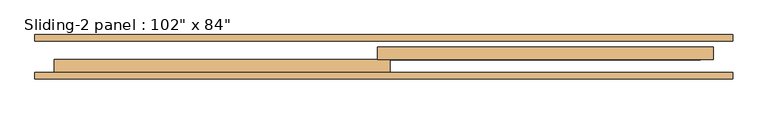
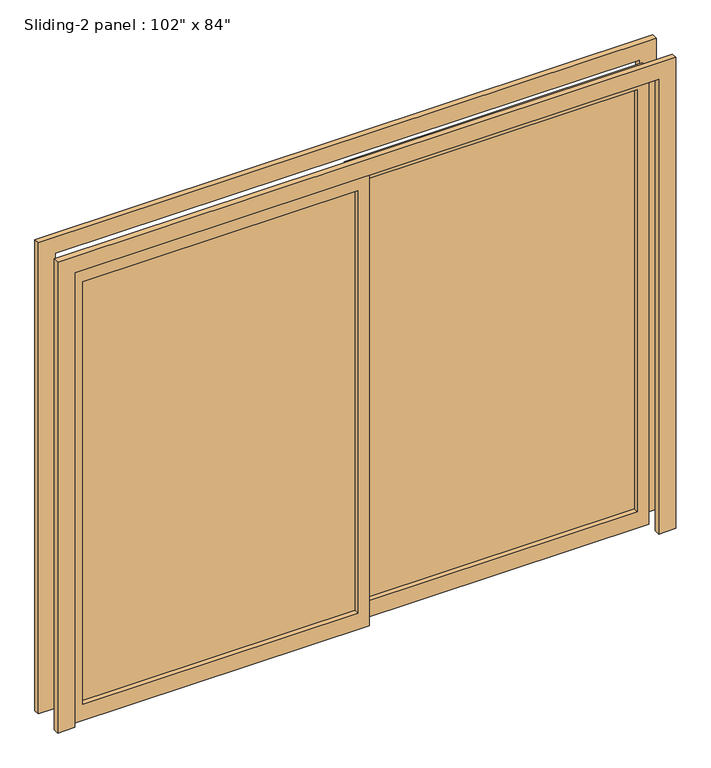
"""IFC4 building model written with IfcOpenShell, lengths in millimetres: door geometry."""

from ifc_helpers import new_model, si_unit, frame, origin, place, context, project, spatial, polyline, outline, extrude, source, transform, mapped, element, save


def door_877872b5(model_context):
    return source(origin(), model_context, "Body", "SweptSolid", [
        extrude(outline(polyline([(25.4, -115.8875), (25.4, -109.5375), (1244.6, -109.5375), (1244.6, -115.8875), (25.4, -115.8875)])), frame((0.0, 0.0, 76.2), z_axis=(0.0, 0.0, 1.0), x_axis=(1.0, 0.0, 0.0)), (0.0, 0.0, 1.0), 1981.2),
        extrude(outline(polyline([(2133.6, -25.4), (0.0, -25.4), (0.0, 1295.4), (2133.6, 1295.4), (2133.6, -25.4)]), holes=[polyline([(2057.4, 25.4), (2057.4, 1244.6), (76.2, 1244.6), (76.2, 25.4), (2057.4, 25.4)])]), frame((0.0, -138.1125, 0.0), z_axis=(0.0, 1.0, 0.0), x_axis=(0.0, 0.0, 1.0)), (0.0, 0.0, 1.0), 50.8),
        extrude(outline(polyline([(-1244.6, -166.6875), (-1244.6, -160.3375), (-25.4, -160.3375), (-25.4, -166.6875), (-1244.6, -166.6875)])), frame((0.0, 0.0, 76.2), z_axis=(0.0, 0.0, 1.0), x_axis=(1.0, 0.0, 0.0)), (0.0, 0.0, 1.0), 1981.2),
        extrude(outline(polyline([(2133.6, 25.4), (2133.6, -1295.4), (0.0, -1295.4), (0.0, 25.4), (2133.6, 25.4)]), holes=[polyline([(2057.4, -25.4), (76.2, -25.4), (76.2, -1244.6), (2057.4, -1244.6), (2057.4, -25.4)])]), frame((0.0, -188.9125, 0.0), z_axis=(0.0, 1.0, 0.0), x_axis=(0.0, 0.0, 1.0)), (0.0, 0.0, 1.0), 50.8),
        extrude(outline(polyline([(0.0, -1371.6), (0.0, -1295.4), (2133.6, -1295.4), (2133.6, 1295.4), (0.0, 1295.4), (0.0, 1371.6), (2209.8, 1371.6), (2209.8, -1371.6), (0.0, -1371.6)])), frame((0.0, -65.0875, 0.0), z_axis=(0.0, 1.0, 0.0), x_axis=(0.0, 0.0, 1.0)), (0.0, 0.0, 1.0), 25.4),
        extrude(outline(polyline([(0.0, 1371.6), (2209.8, 1371.6), (2209.8, -1371.6), (0.0, -1371.6), (0.0, -1295.4), (2133.6, -1295.4), (2133.6, 1295.4), (0.0, 1295.4), (0.0, 1371.6)])), frame((0.0, -214.3125, 0.0), z_axis=(0.0, 1.0, 0.0), x_axis=(0.0, 0.0, 1.0)), (0.0, 0.0, 1.0), 25.4),
    ])


if __name__ == "__main__":
    model = new_model("IFC4")
    model_context = context("Model", 3, world=origin())
    ifc_project = project(units=[si_unit("LENGTHUNIT", "METRE", prefix="MILLI")], contexts=[model_context])
    site = spatial("IfcSite", under=ifc_project)
    building = spatial("IfcBuilding", under=site)
    placement = place(None, origin())
    door_shape = door_877872b5(model_context)
    element("IfcDoor", 1, ObjectType="Sliding-2 panel : 102\" x 84\"", at=placement, inside=building, context=model_context, shape_type="MappedRepresentation", body=[
        mapped(door_shape, transform((0.0, 0.0, 0.0), x_axis=(1.0, 0.0, 0.0), y_axis=(0.0, 1.0, 0.0), z_axis=(0.0, 0.0, 1.0))),
    ])
    save(model, "model.ifc")

# Revit data of these elements
# Type "Sliding-2 panel : 102\" x 84\""
#   Type Mark = "24"
#   Assembly Code = "C1020"
#   Thickness = 0' - 2"
#   Height = 7' - 0"
#   Rail Width = 0' - 3"
#   Stile Width = 0' - 2"
#   Trim Projection Ext = 0' - 1"
#   Trim Projection Int = 0' - 1"
#   Trim Width = 0' - 3"
#   Width = 8' - 6"
#   Door Material = Door - Panel
#   Frame Material = Door - Frame
#   Function = (empty or 0)
#   Wall Closure = (empty or 0)
# Element 1 (IfcDoor, "Sliding-2 panel : 102\" x 84\"")
#   Materials on its faces: "Door - Panel", "Door - Frame", "Glass"
# Materials
#   "Door - Panel": class "Wood", colour RGB 210 159 95, transparency 0
#   "Door - Frame": class "Miscellaneous", colour RGB 118 70 51, transparency 0
#   "Glass": class "Glass", colour RGB 0 128 192, transparency 0.75
